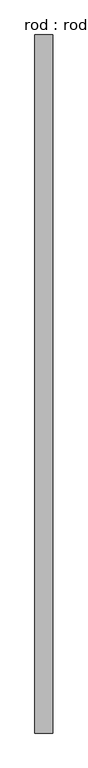
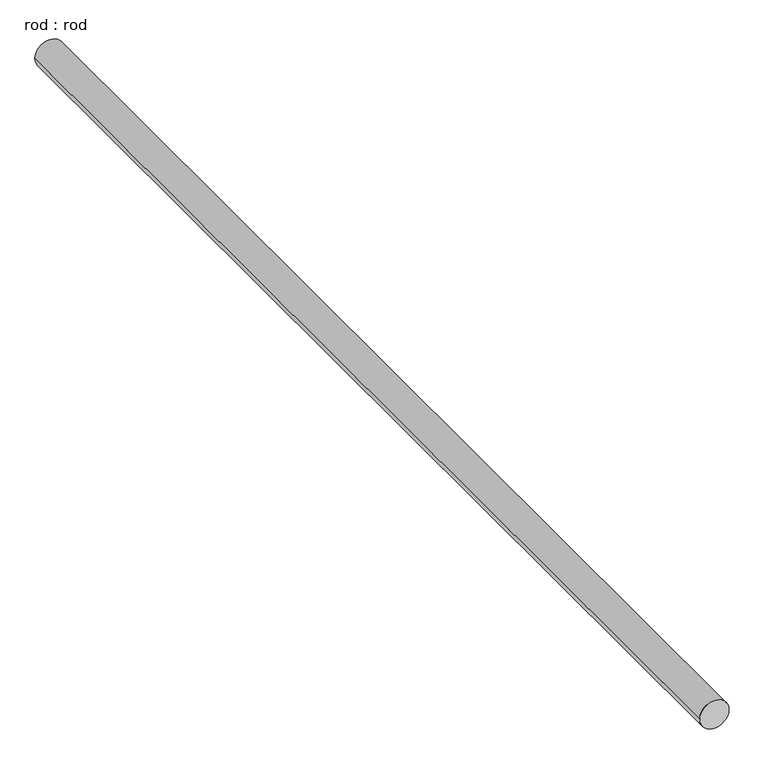
"""IFC4 building model written with IfcOpenShell, lengths in millimetres: proxy geometry, rod : rod."""

from ifc_helpers import new_model, si_unit, point, frame, frame_2d, origin, place, context, project, spatial, circle_curve, trimmed, segment, composite_curve, outline, extrude, source, transform, mapped, element, save


def rod_rod_93cef763(model_context):
    return source(origin(), model_context, "Body", "SweptSolid", [
        extrude(outline(composite_curve([segment(trimmed(circle_curve(frame_2d((0.0108462, 0.0)), 200.0), [point((0.0108462, 200.0))], [point((0.0108462, -200.0))], False, "CARTESIAN"), True, "CONTINUOUS"), segment(trimmed(circle_curve(frame_2d((0.0108462, 0.0)), 200.0), [point((0.0108462, -200.0))], [point((0.0108462, 200.0))], False, "CARTESIAN"), True, "CONTINUOUS")], self_intersect=False)), frame((0.0, -3780.3904036, 0.0), z_axis=(0.0, 1.0, 0.0), x_axis=(0.0, 0.0, 1.0)), (0.0, 0.0, 1.0), 15746.2380379),
    ])


if __name__ == "__main__":
    model = new_model("IFC4")
    model_context = context("Model", 3, world=origin())
    ifc_project = project(units=[si_unit("LENGTHUNIT", "METRE", prefix="MILLI")], contexts=[model_context])
    site = spatial("IfcSite", under=ifc_project)
    building = spatial("IfcBuilding", under=site)
    placement = place(None, origin())
    rod_rod_shape = rod_rod_93cef763(model_context)
    element("IfcBuildingElementProxy", 1, Name="rod : rod", ObjectType="rod : rod", at=placement, inside=building, context=model_context, shape_type="MappedRepresentation", body=[
        mapped(rod_rod_shape, transform((0.0, 0.0, 0.0), x_axis=(1.0, 0.0, 0.0), y_axis=(0.0, 1.0, 0.0), z_axis=(0.0, 0.0, 1.0))),
    ])
    save(model, "model.ifc")

# Revit data of these elements
# Type "rod : rod"
#   Default Elevation = 0
